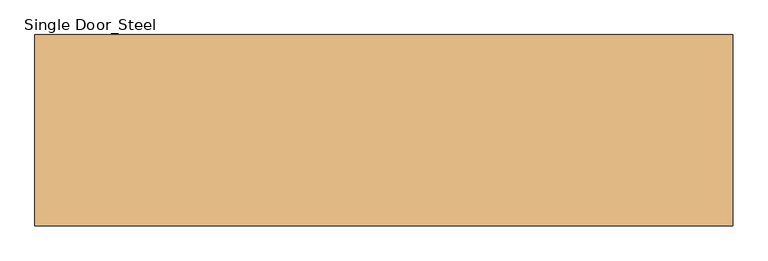
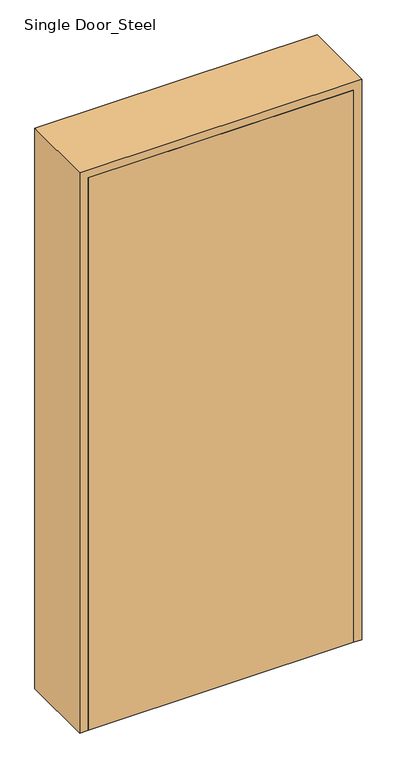
"""IFC4 building model written with IfcOpenShell, lengths in millimetres: door geometry, Single Door_Steel : H_DR_AMD_Single Door_Int_Steel_1000x2100."""

from ifc_helpers import new_model, si_unit, origin, origin_with_axes, place, context, project, spatial, polyline, outline, extrude, faceted_brep, source, transform, mapped, element, save


def single_door_steel_c730d40a(model_context):
    return source(origin(), model_context, "Body", "SolidModel", [
        extrude(outline(polyline([(470.0, -137.0), (-470.0, -137.0), (-470.0, -102.0), (470.0, -102.0), (470.0, -137.0)])), origin_with_axes(), (0.0, 0.0, 1.0), 2070.0),
        faceted_brep([(470.0, -137.0, 0.0), (470.0, -102.0, 0.0), (450.0, -102.0, 0.0), (450.0, 102.0, 0.0), (470.0, 102.0, 0.0), (470.0, 137.0, 0.0), (500.0, 137.0, 0.0), (500.0, -137.0, 0.0), (500.0, -137.0, 2100.0), (-500.0, -137.0, 2100.0), (-500.0, -137.0, 0.0), (-470.0, -137.0, 0.0), (-470.0, -137.0, 2070.0), (470.0, -137.0, 2070.0), (500.0, 137.0, 2100.0), (470.0, 137.0, 2070.0), (-470.0, 137.0, 2070.0), (-470.0, 137.0, 0.0), (-500.0, 137.0, 0.0), (-500.0, 137.0, 2100.0), (470.0, 102.0, 2070.0), (450.0, 102.0, 2050.0), (-450.0, 102.0, 2050.0), (-450.0, 102.0, 0.0), (-470.0, 102.0, 0.0), (-470.0, 102.0, 2070.0), (450.0, -102.0, 2050.0), (470.0, -102.0, 2070.0), (-470.0, -102.0, 2070.0), (-470.0, -102.0, 0.0), (-450.0, -102.0, 0.0), (-450.0, -102.0, 2050.0)], [[[0, 1, 2, 3, 4, 5, 6, 7]], [[7, 8, 9, 10, 11, 12, 13, 0]], [[6, 14, 8, 7]], [[5, 15, 16, 17, 18, 19, 14, 6]], [[4, 20, 15, 5]], [[3, 21, 22, 23, 24, 25, 20, 4]], [[2, 26, 21, 3]], [[1, 27, 28, 29, 30, 31, 26, 2]], [[0, 13, 27, 1]], [[12, 11, 29, 28]], [[11, 10, 18, 17, 24, 23, 30, 29]], [[19, 18, 10, 9]], [[25, 24, 17, 16]], [[31, 30, 23, 22]], [[14, 19, 9, 8]], [[20, 25, 16, 15]], [[26, 31, 22, 21]], [[13, 12, 28, 27]]]),
    ])


if __name__ == "__main__":
    model = new_model("IFC4")
    model_context = context("Model", 3, world=origin())
    ifc_project = project(units=[si_unit("LENGTHUNIT", "METRE", prefix="MILLI")], contexts=[model_context])
    site = spatial("IfcSite", under=ifc_project)
    building = spatial("IfcBuilding", under=site)
    placement = place(None, origin())
    single_door_steel_shape = single_door_steel_c730d40a(model_context)
    element("IfcDoor", 1, ObjectType="Single Door_Steel : H_DR_AMD_Single Door_Int_Steel_1000x2100", at=placement, inside=building, context=model_context, shape_type="MappedRepresentation", body=[
        mapped(single_door_steel_shape, transform((0.0, 0.0, 0.0), x_axis=(1.0, 0.0, 0.0), y_axis=(0.0, 1.0, 0.0), z_axis=(0.0, 0.0, 1.0))),
    ])
    save(model, "model.ifc")

# Revit data of these elements
# Type "Single Door_Steel : H_DR_AMD_Single Door_Int_Steel_1000x2100"
#   Type Mark = "SD"
#   Analytic Construction = "<None>"
#   프레임 투영 외부. = 0.0250 m
#   프레임 투영 내부. = 0.0250 m
#   프레임 폭 = 0.0750 m
#   Height = 2.1000 m
#   Width = 1.0000 m
#   Define Thermal Properties by = 1
#   문 패널 = SD1 문 패널
#   문 프레임 = A04AR099-00001_Steel Door_Single_FR_N
#   Function = (empty or 0)
#   Wall Closure = (empty or 0)
# Element 1 (IfcDoor, "Single Door_Steel : H_DR_AMD_Single Door_Int_Steel_1000x2100")
#   Materials on its faces: "A04AR099-00001_Steel Door_Single_FR_N", "SD1 문 패널"
# Materials
#   "SD1 문 패널": class "금속", colour RGB 247 247 247, transparency 0, Description = "STEEL DOOR (1000Wx2100H)"
#   "A04AR099-00001_Steel Door_Single_FR_N": class "Metal", colour RGB 247 247 247, transparency 0, Description = "Steel Door w/ Steel Frame", Cost = 0
